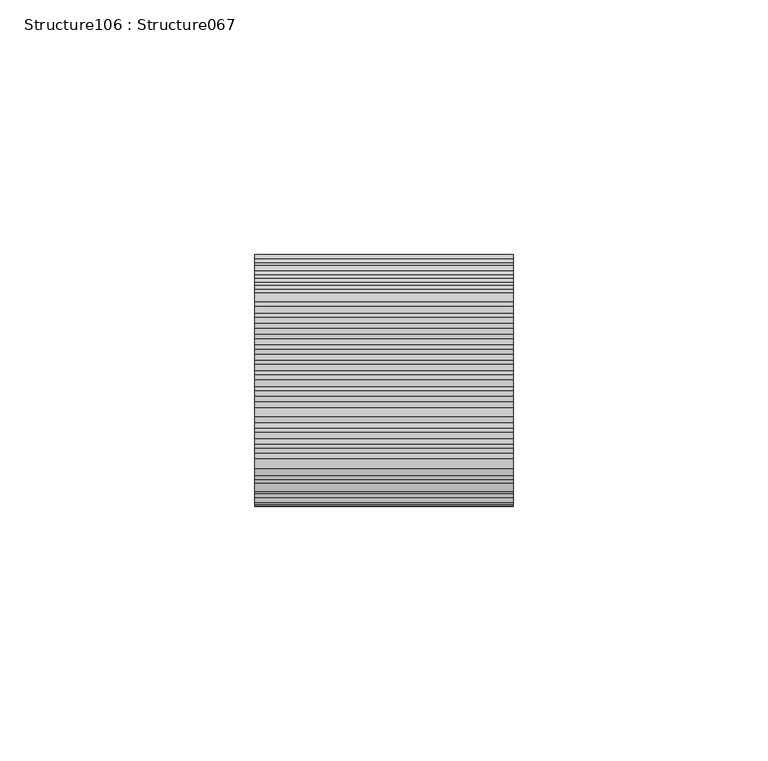
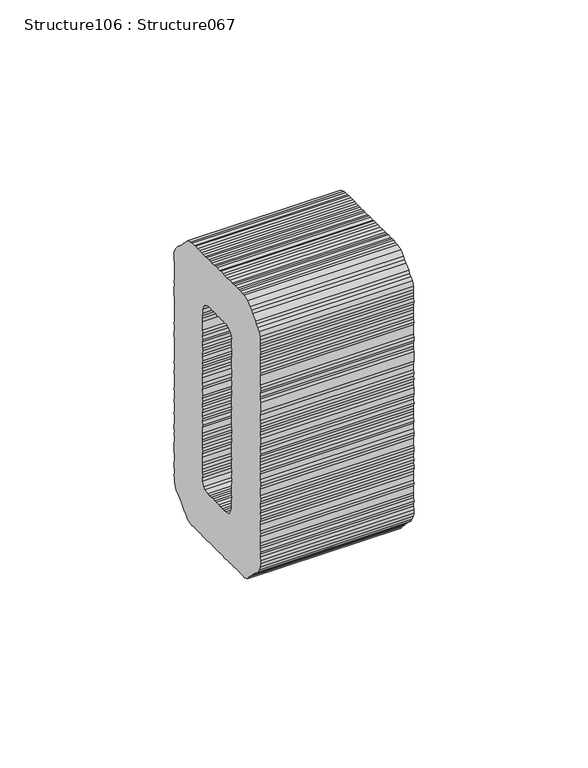
"""IFC4 building model written with IfcOpenShell, lengths in millimetres: proxy geometry, Structure106 : Structure067."""

import ifcopenshell
import ifcopenshell.guid

model = None  # the IFC model being written
_history = None  # IfcOwnerHistory: only IFC2X3 demands one
_inside = {}  # id of a spatial element -> (the spatial element, [elements in it])
_under = {}  # id of a project, library or spatial element -> (it, [spatial elements below it])
_declared = {}  # id of a project -> (the project, [libraries it declares])
_typed = {}  # id of a type object -> (the type object, [elements of that type])
_made_of = {}  # id of a material, layer set ... -> (it, [elements and type objects made of it])


def new_model(schema):
    """Start an empty IFC model of exactly this schema.

    Asked for "IFC4X3", IfcOpenShell would pick the latest addendum, in which some entities
    have other attributes; the version numbers below select the first issue.
    IFC2X3 requires an IfcOwnerHistory on every rooted entity: one is made here for all.
    """
    global model, _history
    if schema == "IFC4X3":
        model = ifcopenshell.file(schema_version=(4, 3, 0, 0))
    else:
        model = ifcopenshell.file(schema=schema)
    _inside.clear()
    _under.clear()
    _declared.clear()
    _typed.clear()
    _made_of.clear()
    _history = None
    if model.schema == "IFC2X3":
        org = make("IfcOrganization", Name="unknown")
        user = make(
            "IfcPersonAndOrganization",
            ThePerson=make("IfcPerson", FamilyName="unknown"),
            TheOrganization=org,
        )
        app = make(
            "IfcApplication",
            ApplicationDeveloper=org,
            Version="unknown",
            ApplicationFullName="unknown",
            ApplicationIdentifier="unknown",
        )
        _history = make(
            "IfcOwnerHistory",
            OwningUser=user,
            OwningApplication=app,
            ChangeAction="ADDED",
            CreationDate=0,
        )
    return model


def make(cls, **values):
    """One entity of the class cls with the attributes given. An attribute that is None is left unset."""
    return model.create_entity(
        cls, **{name: value for name, value in values.items() if value is not None}
    )


def rooted(cls, **values):
    """An entity with a GlobalId (a new one), such as an element, a storey or a relation."""
    return make(cls, GlobalId=ifcopenshell.guid.new(), OwnerHistory=_history, **values)


def si_unit(unit_type, name, prefix=None):
    """IfcSIUnit, for example si_unit("LENGTHUNIT", "METRE", prefix="MILLI")."""
    return make("IfcSIUnit", UnitType=unit_type, Prefix=prefix, Name=name)


def assignment(units):
    """IfcUnitAssignment: the units of a project."""
    return None if units is None else make("IfcUnitAssignment", Units=units)


def point(xyz):
    """IfcCartesianPoint."""
    return None if xyz is None else make("IfcCartesianPoint", Coordinates=xyz)


def direction(xyz):
    """IfcDirection."""
    return None if xyz is None else make("IfcDirection", DirectionRatios=xyz)


def frame(location, z_axis=None, x_axis=None):
    """IfcAxis2Placement3D, a coordinate frame: its origin and axes. An axis left out is left unset."""
    return make(
        "IfcAxis2Placement3D",
        Location=point(location),
        Axis=direction(z_axis),
        RefDirection=direction(x_axis),
    )


def origin():
    """The frame at (0, 0, 0) with its axes left unset."""
    return frame((0.0, 0.0, 0.0))


def place(relative_to, where):
    """IfcLocalPlacement: puts the frame where relative to a parent placement (None: the world)."""
    return make(
        "IfcLocalPlacement", PlacementRelTo=relative_to, RelativePlacement=where
    )


def context(
    kind, dimensions, precision=None, world=None, true_north=None, identifier=None
):
    """IfcGeometricRepresentationContext, for example the 3D "Model" context."""
    return make(
        "IfcGeometricRepresentationContext",
        ContextIdentifier=identifier,
        ContextType=kind,
        CoordinateSpaceDimension=dimensions,
        Precision=precision,
        WorldCoordinateSystem=world,
        TrueNorth=true_north,
    )


def project(units=None, contexts=None):
    """IfcProject with its units and contexts."""
    return rooted(
        "IfcProject",
        Name="project",
        RepresentationContexts=contexts,
        UnitsInContext=assignment(units),
    )


def spatial(cls, under=None, at=None, **own):
    """A site, building, storey or space (cls), placed at a placement, below another one or the project."""
    s = rooted(cls, ObjectPlacement=at, **own)
    if under is not None:
        _under.setdefault(under.id(), (under, []))[1].append(s)
    return s


def polyline(points):
    """IfcPolyline through the points."""
    return make("IfcPolyline", Points=[point(p) for p in points])


def outline(outer, holes=None, kind="AREA"):
    """IfcArbitraryClosedProfileDef: a profile drawn as a closed curve; with holes, ...WithVoids."""
    if holes is None:
        return make("IfcArbitraryClosedProfileDef", ProfileType=kind, OuterCurve=outer)
    return make(
        "IfcArbitraryProfileDefWithVoids",
        ProfileType=kind,
        OuterCurve=outer,
        InnerCurves=holes,
    )


def extrude(swept, where, along, depth):
    """IfcExtrudedAreaSolid: the profile swept, set in the frame where, extruded along a direction by depth."""
    return make(
        "IfcExtrudedAreaSolid",
        SweptArea=swept,
        Position=where,
        ExtrudedDirection=direction(along),
        Depth=depth,
    )


def shape(context_of_items, identifier, shape_type, items):
    """IfcShapeRepresentation: the items that make up one representation, for example the "Body"."""
    return make(
        "IfcShapeRepresentation",
        ContextOfItems=context_of_items,
        RepresentationIdentifier=identifier,
        RepresentationType=shape_type,
        Items=items,
    )


def source(mapping_origin, context_of_items, identifier, shape_type, items):
    """IfcRepresentationMap: a shape defined once, which mapped items show again and again."""
    return make(
        "IfcRepresentationMap",
        MappingOrigin=mapping_origin,
        MappedRepresentation=shape(context_of_items, identifier, shape_type, items),
    )


def transform(
    local_origin,
    x_axis=None,
    y_axis=None,
    z_axis=None,
    scale=None,
    scale2=None,
    scale3=None,
    uniform=True,
):
    """IfcCartesianTransformationOperator3D, or its non-uniform kind. x_axis, y_axis, z_axis: its Axis1, 2, 3."""
    if uniform:
        return make(
            "IfcCartesianTransformationOperator3D",
            Axis1=direction(x_axis),
            Axis2=direction(y_axis),
            LocalOrigin=point(local_origin),
            Scale=scale,
            Axis3=direction(z_axis),
        )
    return make(
        "IfcCartesianTransformationOperator3DnonUniform",
        Axis1=direction(x_axis),
        Axis2=direction(y_axis),
        LocalOrigin=point(local_origin),
        Scale=scale,
        Axis3=direction(z_axis),
        Scale2=scale2,
        Scale3=scale3,
    )


def mapped(mapping_source, mapping_target):
    """IfcMappedItem: shows the shape of a source again, moved by a transform."""
    return make(
        "IfcMappedItem", MappingSource=mapping_source, MappingTarget=mapping_target
    )


def made_of(thing, what):
    """Note that an element or type object is made of a material, layer set ...; save() writes the relation."""
    if what is not None:
        _made_of.setdefault(what.id(), (what, []))[1].append(thing)
    return thing


def element(
    cls,
    number,
    at=None,
    inside=None,
    cuts=None,
    type_object=None,
    material=None,
    context=None,
    identifier="Body",
    shape_type=None,
    held_by="IfcProductDefinitionShape",
    body=None,
    shapes=None,
    **own,
):
    """One element of the class cls, such as IfcWall. Its Tag is "e" and its number.

    at: its placement. inside: the storey or other place that contains it. cuts: it is an
    opening in that element (IfcRelVoidsElement). A single representation is given by context,
    identifier, shape_type and body (its items); several are given by shapes. held_by: the class
    of the entity that holds the representations. save() writes the other relations.
    """
    e = rooted(cls, Tag="e%d" % number, ObjectPlacement=at, **own)
    if body is not None:
        shapes = [shape(context, identifier, shape_type, body)]
    if shapes is not None:
        e.Representation = make(held_by, Representations=shapes)
    if inside is not None:
        _inside.setdefault(inside.id(), (inside, []))[1].append(e)
    if cuts is not None:
        rooted(
            "IfcRelVoidsElement", RelatingBuildingElement=cuts, RelatedOpeningElement=e
        )
    if type_object is not None:
        _typed.setdefault(type_object.id(), (type_object, []))[1].append(e)
    return made_of(e, material)


def aggregate(whole, parts):
    """IfcRelAggregates: a whole, such as a stair, and the parts it consists of."""
    return rooted("IfcRelAggregates", RelatingObject=whole, RelatedObjects=parts)


def save(model, path):
    """Write the relations noted so far, then the file.

    IfcRelAggregates (storeys below a building ...), IfcRelContainedInSpatialStructure (elements
    in a storey), IfcRelDefinesByType, IfcRelAssociatesMaterial and IfcRelDeclares: one each for
    every whole, place, type object, material and project.
    """
    for whole, parts in _under.values():
        aggregate(whole, parts)
    for where, things in _inside.values():
        rooted(
            "IfcRelContainedInSpatialStructure",
            RelatedElements=things,
            RelatingStructure=where,
        )
    for kind, things in _typed.values():
        rooted("IfcRelDefinesByType", RelatedObjects=things, RelatingType=kind)
    for what, things in _made_of.values():
        rooted("IfcRelAssociatesMaterial", RelatedObjects=things, RelatingMaterial=what)
    for by, libraries in _declared.values():
        rooted("IfcRelDeclares", RelatingContext=by, RelatedDefinitions=libraries)
    model.write(path)


def structure106_structure067_5bbbb801(model_context):
    return source(origin(), model_context, "Body", "SweptSolid", [
        extrude(outline(polyline([(1.9860445, 0.0), (2.6789094, -0.7882832), (3.8239592, -1.2173664), (5.3807843, -2.3653471), (6.3497852, -3.2236496), (7.0882407, -3.6107772), (8.0066376, -4.2175769), (9.1528806, -4.65259), (9.8415639, -5.445344), (10.8594989, -7.2214925), (11.1707557, -8.0920017), (11.5266801, -9.2097639), (11.5546014, -9.9997253), (11.6286642, -11.0442649), (12.1416474, -12.266168), (12.3476425, -13.2899692), (12.2954285, -14.3581017), (12.5003006, -15.3763217), (12.8104344, -16.2412497), (13.1408112, -17.2320397), (13.730652, -20.1635644), (13.8103704, -21.2109584), (14.040369, -22.3540577), (14.3966443, -23.4735641), (14.4256885, -24.2691066), (14.781613, -25.3868688), (14.9872571, -26.4089259), (15.0395328, -27.3199295), (15.139845, -28.4949295), (15.3454892, -29.5169867), (15.7807768, -30.3527406), (15.8859726, -31.526758), (16.3216153, -33.6919145), (16.6775398, -34.8096767), (16.7321316, -35.7321914), (16.8312507, -36.9012615), (17.0114174, -37.7966951), (17.4985021, -38.8898819), (17.4210914, -39.8327863), (17.7826714, -40.9534029), (17.8049371, -41.7405098), (18.0616063, -43.0161625), (18.7284366, -45.0026899), (18.7567088, -45.7943953), (18.8558279, -46.9634655), (19.2919577, -47.8034053), (19.2408667, -48.877119), (19.6016747, -49.9938986), (19.6764393, -51.0419265), (20.7011508, -56.1347704), (21.1636002, -57.1055196), (21.3935287, -58.2482701), (21.4218009, -59.0399755), (21.5221131, -60.2149756), (22.0339733, -61.4312976), (21.9577558, -62.3801319), (22.7775952, -66.4547559), (23.138333, -67.5711868), (23.213238, -68.6199123), (23.4180399, -69.6377835), (24.0334943, -71.368971), (24.4953163, -73.664239), (24.5743328, -74.7081449), (24.8784601, -75.5684743), (24.8021724, -76.5169599), (25.1629804, -77.6337395), (25.2126185, -78.556888), (25.5734966, -79.6740165), (25.7528913, -80.5656131), (25.8276559, -81.6136409), (26.5443883, -83.8481827), (26.9297079, -85.7632317), (26.371283, -87.5984982), (25.7853557, -88.6440823), (25.4039477, -89.3802981), (24.5409722, -90.3513281), (23.902899, -91.1395495), (23.3970369, -91.9066133), (22.8107609, -92.9522675), (22.304197, -93.7158432), (21.6937749, -94.6396873), (21.2071753, -95.5295438), (19.5530516, -96.5280079), (18.6869304, -96.8322118), (17.4126729, -97.0886003), (16.6774334, -97.3686475), (15.5294505, -97.5996287), (14.4863806, -97.6773882), (13.338049, -97.9084396), (12.4216748, -97.9628847), (11.2782266, -98.1929535), (10.4068731, -98.4982102), (9.4904989, -98.5526553), (8.3721773, -98.9076035), (7.5817289, -98.9367116), (6.3074715, -99.1931), (5.5669272, -99.472037), (4.5753014, -99.8036708), (3.2503698, -99.8082076), (2.5357219, -100.2140467), (1.3922739, -100.4441155), (0.3443204, -100.5228576), (-0.828789, -100.6289594), (-2.5564244, -101.2386178), (-3.7550813, -101.2177474), (-4.7219295, -101.6743307), (-5.4872514, -101.8283182), (-6.7870565, -101.9577344), (-7.7790312, -102.2894384), (-8.5443531, -102.4434258), (-9.6125495, -102.396306), (-10.6349553, -102.6020203), (-12.6724459, -102.3463317), (-14.3292984, -101.3524044), (-15.2483972, -100.7421164), (-16.0409385, -100.1096308), (-18.0013673, -98.911108), (-18.563423, -98.0965052), (-19.4562021, -97.6170266), (-20.6279926, -97.0550411), (-21.3186987, -95.6010422), (-21.6746231, -94.48328), (-21.9046217, -93.3401807), (-21.9842699, -92.2931354), (-22.1635944, -91.4018877), (-22.626465, -90.4290457), (-22.67491, -89.5118271), (-22.8794312, -88.4953513), (-22.9583774, -87.4517943), (-23.189499, -86.3031138), (-23.5461955, -85.1815144), (-23.6250716, -84.1383062), (-24.0611313, -83.2987152), (-24.0101104, -82.2246527), (-24.6505551, -79.0416252), (-25.0854918, -78.2076155), (-25.3166134, -77.0589349), (-25.340002, -76.266247), (-25.5962501, -74.9926871), (-25.649719, -74.0757535), (-26.0857787, -73.2361625), (-26.7262233, -70.0531351), (-26.7258064, -68.7275697), (-27.1099328, -66.8184509), (-27.5468347, -65.974674), (-27.6715014, -64.6786316), (-27.9565789, -63.9382341), (-28.0314138, -62.8898573), (-28.2358647, -61.8737304), (-28.5727394, -60.8759), (-28.9808693, -58.847483), (-29.0556339, -57.7994552), (-29.2605762, -56.7808864), (-29.6476336, -55.5336463), (-29.6973419, -54.6101489), (-29.9017929, -53.5940218), (-29.9818622, -52.5448836), (-30.1856113, -51.5322449), (-30.5422376, -50.4109944), (-30.879042, -49.4135129), (-30.8005084, -48.4761896), (-31.1855473, -46.5625361), (-31.6722108, -45.4714423), (-31.8527285, -44.5742647), (-31.9519177, -43.4048457), (-32.4130379, -41.1130659), (-32.7231718, -40.2481379), (-32.9280439, -39.2299179), (-33.0028787, -38.1815412), (-33.1080744, -37.0075237), (-33.5430111, -36.1735138), (-33.5173975, -34.9731767), (-33.9279798, -34.2602091), (-34.1336239, -33.2381521), (-34.1072383, -32.041652), (-34.4125588, -31.1753925), (-34.8481314, -29.010585), (-35.1571423, -28.1512381), (-35.232328, -27.1011173), (-35.6930972, -24.8110817), (-35.7731665, -23.7619435), (-35.952491, -22.8706958), (-36.4137474, -21.9058766), (-36.4622625, -20.9883093), (-36.5419808, -19.9409152), (-37.0035881, -18.9743519), (-37.2335867, -17.8312526), (-37.3338989, -16.6562525), (-36.8766221, -14.9712725), (-36.4462118, -13.8274074), (-35.8096105, -13.0336751), (-35.3026976, -12.2700292), (-34.6660964, -11.4762968), (-33.9527014, -10.4112356), (-33.4723869, -9.5171994), (-32.3486946, -7.8360522), (-31.8935767, -6.8167878), (-30.2394531, -5.8183238), (-29.0648018, -5.7180817), (-28.022153, -5.6382293), (-27.1560318, -5.3340255), (-26.2393088, -5.2795101), (-25.1209872, -4.924562), (-24.224856, -4.7442549), (-22.925472, -4.6127457), (-22.1901602, -4.3348616), (-21.016702, -4.2286895), (-20.1765515, -3.7936062), (-19.1593781, -3.5889446), (-18.0855261, -3.6389189), (-17.1942784, -3.4595944), (-16.0759567, -3.1046463), (-13.0139716, -2.4885561), (-11.9762063, -2.4096862), (-10.9541493, -2.2040421), (-9.9880731, -1.7436217), (-9.0968254, -1.5642972), (-8.1740257, -1.5147293), (-7.0568972, -1.1538512), (-5.8574683, -1.1785586), (-4.9909982, -0.8742846), (-3.9734759, -0.6695529), (-2.8003666, -0.563451), (-1.7828443, -0.3587192), (-0.9167231, -0.0545154), (0.0, 0.0), (1.9860445, 0.0)]), holes=[polyline([(-6.2250852, -83.6817193), (-3.6710508, -84.4987576), (-2.679074, -84.1688678), (-1.7622808, -84.1147013), (-0.7961345, -83.6546297), (0.2772986, -83.7043254), (1.243445, -83.2442538), (2.3119943, -83.2949321), (3.3295167, -83.0902004), (4.4526517, -82.7339208), (5.3690961, -82.6798245), (6.3915019, -82.4741102), (8.0156155, -81.3517493), (8.4004354, -80.6090398), (8.7534309, -79.0804209), (8.4971828, -77.806861), (8.5491161, -76.7373332), (8.2437956, -75.8710738), (8.1385998, -74.6970562), (7.5247555, -71.6462334), (7.1130503, -70.9276846), (7.1143095, -69.6063052), (6.652632, -68.6393932), (6.6296644, -67.8487981), (6.4989211, -66.5478083), (6.0620894, -65.7043802), (5.8835369, -64.8169696), (5.884024, -63.4917531), (5.7034362, -62.5942265), (5.2167726, -61.5031327), (5.1430608, -60.4603373), (4.8580534, -59.7202885), (4.809468, -58.8023724), (4.4730847, -57.8069838), (4.4998915, -56.6125766), (4.1438969, -55.4944656), (3.7589282, -53.5811609), (3.4232468, -52.5892605), (3.4488604, -51.3889234), (2.7816791, -49.4006518), (2.8338931, -48.3325193), (2.4240829, -47.6233888), (2.3237707, -46.4483887), (2.270372, -45.531804), (1.8079927, -44.5614036), (1.7339299, -43.516864), (1.4776818, -42.2433042), (1.1930254, -41.5049995), (1.2448885, -40.4351229), (0.7581547, -39.3436803), (0.734766, -38.5509923), (0.2984214, -36.3823478), (0.2194751, -35.3387907), (-0.0105235, -34.1956914), (-0.2906473, -33.4546601), (-0.3947201, -32.2862238), (-0.7251671, -31.295085), (-1.0364239, -30.4245757), (-0.9845609, -29.3546991), (-1.3412573, -28.2330997), (-1.7254539, -26.3236321), (-1.8051723, -25.276238), (-2.1610967, -24.1584758), (-2.3914462, -23.0136324), (-2.6772256, -22.2697466), (-2.650489, -21.0749906), (-3.0064135, -19.9572284), (-3.9549756, -18.5511193), (-4.6960006, -18.1746711), (-6.5508848, -18.1500956), (-7.4688009, -18.198681), (-8.3600486, -18.3780055), (-9.4820606, -18.7398662), (-10.399628, -18.7883814), (-11.3908307, -19.1239225), (-12.6914077, -19.2495015), (-13.4822071, -19.2768656), (-14.7309872, -19.6598774), (-15.6480611, -19.7126487), (-16.7442469, -20.2010627), (-18.3242417, -20.9167569), (-19.0065696, -23.4386056), (-18.8272451, -24.3298533), (-18.4713207, -25.4476155), (-18.2908031, -26.3447931), (-18.3378528, -27.4133385), (-17.9819283, -28.5311007), (-17.8017616, -29.4265343), (-17.4710339, -30.4190684), (-17.2916392, -31.3106649), (-17.2872428, -32.6348988), (-17.0823707, -33.6531187), (-16.7515727, -34.6460017), (-16.6719246, -35.6930469), (-16.4925299, -36.5846434), (-16.1359036, -37.705894), (-15.6509077, -39.4651452), (-15.6982381, -40.5322951), (-15.3423137, -41.6500574), (-15.0359404, -42.5215492), (-14.8576687, -43.4075646), (-14.7269955, -44.7082055), (-14.4209732, -45.5779532), (-14.4428262, -46.7717266), (-14.288558, -47.5384439), (-13.8322554, -48.5038967), (-13.8792349, -49.5727908), (-13.6218639, -50.8519318), (-13.1651401, -51.8194777), (-12.9606189, -52.8359536), (-12.9323467, -53.627659), (-12.5764223, -54.7454212), (-12.4967742, -55.7924665), (-12.291902, -56.8106865), (-12.2133067, -57.8524993), (-11.8554873, -58.9796798), (-11.4724838, -60.8832175), (-11.1660403, -61.7550582), (-11.1878934, -62.9488315), (-11.0073757, -63.8460093), (-10.5773225, -64.6810016), (-10.6243722, -65.7495469), (-10.4186579, -66.7719528), (-9.9368778, -67.8640292), (-9.9576079, -69.0633837), (-9.5470916, -71.1036607), (-9.2673889, -71.8425991), (-8.8579254, -73.8776437), (-8.5260747, -74.8757591), (-8.5479278, -76.0695324), (-8.1378326, -78.1077164), (-7.6555613, -79.2022346), (-7.2969123, -80.98473), (-7.3442427, -82.0518799), (-6.2250852, -83.6817193)])]), frame((-56111.4541329, 291410.5753176, -375.2105814), z_axis=(-0.9999998917542984, 0.0004652863545059616, 0.0), x_axis=(0.00045614469840443234, 0.9803525175672692, 0.19725296761146935)), (0.0, 0.0, 1.0), 50.8),
    ])


if __name__ == "__main__":
    model = new_model("IFC4")
    model_context = context("Model", 3, world=origin())
    ifc_project = project(units=[si_unit("LENGTHUNIT", "METRE", prefix="MILLI")], contexts=[model_context])
    site = spatial("IfcSite", under=ifc_project)
    building = spatial("IfcBuilding", under=site)
    placement = place(None, origin())
    structure106_structure067_shape = structure106_structure067_5bbbb801(model_context)
    element("IfcBuildingElementProxy", 1, Name="Structure106 : Structure067", ObjectType="Structure106 : Structure067", at=placement, inside=building, context=model_context, shape_type="MappedRepresentation", body=[
        mapped(structure106_structure067_shape, transform((0.0, 0.0, 0.0), x_axis=(1.0, 0.0, 0.0), y_axis=(0.0, 1.0, 0.0), z_axis=(0.0, 0.0, 1.0))),
    ])
    save(model, "model.ifc")

# Revit data of these elements
# Type "Structure106 : Structure067"
#   NameOverride = "Structure067"
# Element 1 (IfcBuildingElementProxy, "Structure106 : Structure067")
#   Materials on its faces: "BRUSHED ALUMINUM LETTERING"
# Materials
#   "BRUSHED ALUMINUM LETTERING": class "Unassigned", colour RGB 169 181 186, transparency 0, Cost = 0
